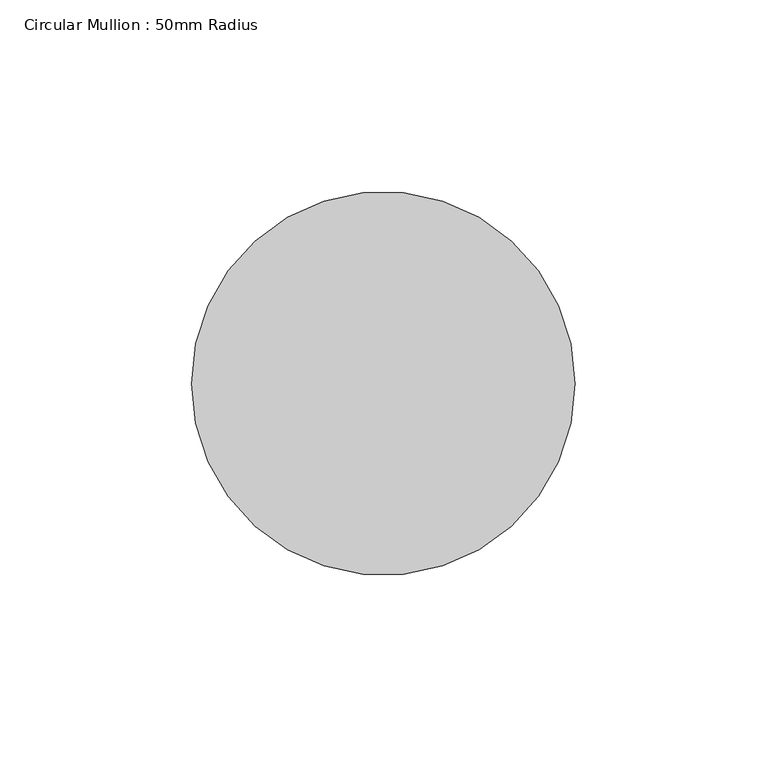
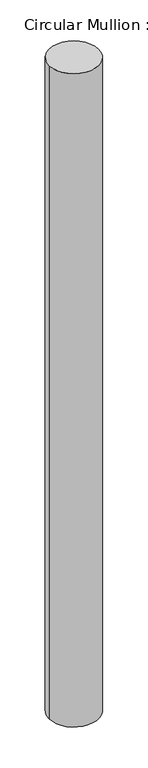
"""IFC4 building model written with IfcOpenShell, lengths in millimetres: member geometry, Circular Mullion : 50mm Radius."""

from ifc_helpers import new_model, si_unit, point, frame, origin, origin_2d, place, context, project, spatial, circle_curve, trimmed, segment, composite_curve, outline, extrude, source, transform, mapped, element, save


def circular_mullion_50mm_radius_0e5e2bfd(model_context):
    return source(origin(), model_context, "Body", "SweptSolid", [
        extrude(outline(composite_curve([segment(trimmed(circle_curve(origin_2d(), 50.0), [point((50.0, 0.0))], [point((-50.0, 0.0))], False, "CARTESIAN"), True, "CONTINUOUS"), segment(trimmed(circle_curve(origin_2d(), 50.0), [point((-50.0, 0.0))], [point((50.0, 0.0))], False, "CARTESIAN"), True, "CONTINUOUS")], self_intersect=False)), frame((0.0, 0.0, -1391.9380385), z_axis=(0.0, 0.0, 1.0), x_axis=(1.0, 0.0, 0.0)), (0.0, 0.0, 1.0), 1391.9380385),
    ])


if __name__ == "__main__":
    model = new_model("IFC4")
    model_context = context("Model", 3, world=origin())
    ifc_project = project(units=[si_unit("LENGTHUNIT", "METRE", prefix="MILLI")], contexts=[model_context])
    site = spatial("IfcSite", under=ifc_project)
    building = spatial("IfcBuilding", under=site)
    placement = place(None, origin())
    circular_mullion_50mm_radius_shape = circular_mullion_50mm_radius_0e5e2bfd(model_context)
    element("IfcMember", 1, ObjectType="Circular Mullion : 50mm Radius", at=placement, inside=building, context=model_context, shape_type="MappedRepresentation", body=[
        mapped(circular_mullion_50mm_radius_shape, transform((0.0, 0.0, 0.0), x_axis=(1.0, 0.0, 0.0), y_axis=(0.0, 1.0, 0.0), z_axis=(0.0, 0.0, 1.0))),
    ])
    save(model, "model.ifc")

# Revit data of these elements
# Type "Circular Mullion : 50mm Radius"
#   built-in parameter 1007350 = 0.164042 (stored number, unit not read)
# Element 1 (IfcMember, "Circular Mullion : 50mm Radius")
#   Materials on its faces: "Aluminium"
# Materials
#   "Aluminium": class "Metal", colour RGB 247 247 247, transparency 0, Description = "Aluminium 6061", Cost = 0
